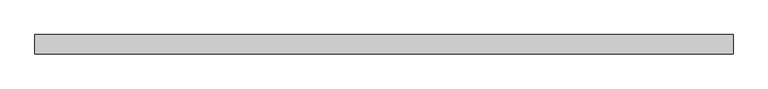
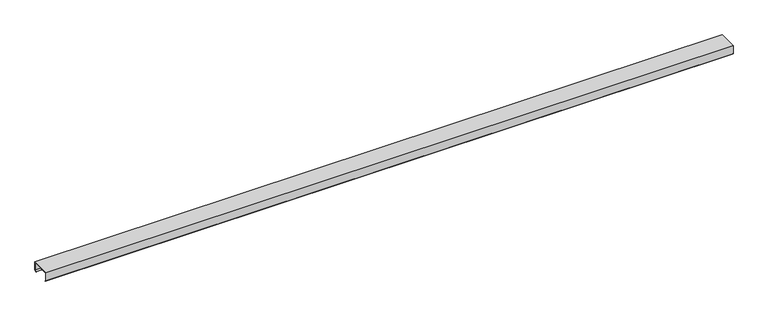
"""IFC4 building model written with IfcOpenShell, lengths in millimetres: proxy geometry, Generic Models 7:Generic Models 1:1:Generic Models 1:1 : Generic Models 7:Generic Models 1:337419:8 : Generic Models 7:Generic Models 1:1:Generic Models 1:1 : Generic Models 7:Generic Models 1:337419:306201."""

import ifcopenshell
import ifcopenshell.guid

model = None  # the IFC model being written
_history = None  # IfcOwnerHistory: only IFC2X3 demands one
_inside = {}  # id of a spatial element -> (the spatial element, [elements in it])
_under = {}  # id of a project, library or spatial element -> (it, [spatial elements below it])
_declared = {}  # id of a project -> (the project, [libraries it declares])
_typed = {}  # id of a type object -> (the type object, [elements of that type])
_made_of = {}  # id of a material, layer set ... -> (it, [elements and type objects made of it])


def new_model(schema):
    """Start an empty IFC model of exactly this schema.

    Asked for "IFC4X3", IfcOpenShell would pick the latest addendum, in which some entities
    have other attributes; the version numbers below select the first issue.
    IFC2X3 requires an IfcOwnerHistory on every rooted entity: one is made here for all.
    """
    global model, _history
    if schema == "IFC4X3":
        model = ifcopenshell.file(schema_version=(4, 3, 0, 0))
    else:
        model = ifcopenshell.file(schema=schema)
    _inside.clear()
    _under.clear()
    _declared.clear()
    _typed.clear()
    _made_of.clear()
    _history = None
    if model.schema == "IFC2X3":
        org = make("IfcOrganization", Name="unknown")
        user = make(
            "IfcPersonAndOrganization",
            ThePerson=make("IfcPerson", FamilyName="unknown"),
            TheOrganization=org,
        )
        app = make(
            "IfcApplication",
            ApplicationDeveloper=org,
            Version="unknown",
            ApplicationFullName="unknown",
            ApplicationIdentifier="unknown",
        )
        _history = make(
            "IfcOwnerHistory",
            OwningUser=user,
            OwningApplication=app,
            ChangeAction="ADDED",
            CreationDate=0,
        )
    return model


def make(cls, **values):
    """One entity of the class cls with the attributes given. An attribute that is None is left unset."""
    return model.create_entity(
        cls, **{name: value for name, value in values.items() if value is not None}
    )


def rooted(cls, **values):
    """An entity with a GlobalId (a new one), such as an element, a storey or a relation."""
    return make(cls, GlobalId=ifcopenshell.guid.new(), OwnerHistory=_history, **values)


def si_unit(unit_type, name, prefix=None):
    """IfcSIUnit, for example si_unit("LENGTHUNIT", "METRE", prefix="MILLI")."""
    return make("IfcSIUnit", UnitType=unit_type, Prefix=prefix, Name=name)


def assignment(units):
    """IfcUnitAssignment: the units of a project."""
    return None if units is None else make("IfcUnitAssignment", Units=units)


def point(xyz):
    """IfcCartesianPoint."""
    return None if xyz is None else make("IfcCartesianPoint", Coordinates=xyz)


def direction(xyz):
    """IfcDirection."""
    return None if xyz is None else make("IfcDirection", DirectionRatios=xyz)


def frame(location, z_axis=None, x_axis=None):
    """IfcAxis2Placement3D, a coordinate frame: its origin and axes. An axis left out is left unset."""
    return make(
        "IfcAxis2Placement3D",
        Location=point(location),
        Axis=direction(z_axis),
        RefDirection=direction(x_axis),
    )


def origin():
    """The frame at (0, 0, 0) with its axes left unset."""
    return frame((0.0, 0.0, 0.0))


def place(relative_to, where):
    """IfcLocalPlacement: puts the frame where relative to a parent placement (None: the world)."""
    return make(
        "IfcLocalPlacement", PlacementRelTo=relative_to, RelativePlacement=where
    )


def context(
    kind, dimensions, precision=None, world=None, true_north=None, identifier=None
):
    """IfcGeometricRepresentationContext, for example the 3D "Model" context."""
    return make(
        "IfcGeometricRepresentationContext",
        ContextIdentifier=identifier,
        ContextType=kind,
        CoordinateSpaceDimension=dimensions,
        Precision=precision,
        WorldCoordinateSystem=world,
        TrueNorth=true_north,
    )


def project(units=None, contexts=None):
    """IfcProject with its units and contexts."""
    return rooted(
        "IfcProject",
        Name="project",
        RepresentationContexts=contexts,
        UnitsInContext=assignment(units),
    )


def spatial(cls, under=None, at=None, **own):
    """A site, building, storey or space (cls), placed at a placement, below another one or the project."""
    s = rooted(cls, ObjectPlacement=at, **own)
    if under is not None:
        _under.setdefault(under.id(), (under, []))[1].append(s)
    return s


def polyline(points):
    """IfcPolyline through the points."""
    return make("IfcPolyline", Points=[point(p) for p in points])


def outline(outer, holes=None, kind="AREA"):
    """IfcArbitraryClosedProfileDef: a profile drawn as a closed curve; with holes, ...WithVoids."""
    if holes is None:
        return make("IfcArbitraryClosedProfileDef", ProfileType=kind, OuterCurve=outer)
    return make(
        "IfcArbitraryProfileDefWithVoids",
        ProfileType=kind,
        OuterCurve=outer,
        InnerCurves=holes,
    )


def extrude(swept, where, along, depth):
    """IfcExtrudedAreaSolid: the profile swept, set in the frame where, extruded along a direction by depth."""
    return make(
        "IfcExtrudedAreaSolid",
        SweptArea=swept,
        Position=where,
        ExtrudedDirection=direction(along),
        Depth=depth,
    )


def shape(context_of_items, identifier, shape_type, items):
    """IfcShapeRepresentation: the items that make up one representation, for example the "Body"."""
    return make(
        "IfcShapeRepresentation",
        ContextOfItems=context_of_items,
        RepresentationIdentifier=identifier,
        RepresentationType=shape_type,
        Items=items,
    )


def source(mapping_origin, context_of_items, identifier, shape_type, items):
    """IfcRepresentationMap: a shape defined once, which mapped items show again and again."""
    return make(
        "IfcRepresentationMap",
        MappingOrigin=mapping_origin,
        MappedRepresentation=shape(context_of_items, identifier, shape_type, items),
    )


def transform(
    local_origin,
    x_axis=None,
    y_axis=None,
    z_axis=None,
    scale=None,
    scale2=None,
    scale3=None,
    uniform=True,
):
    """IfcCartesianTransformationOperator3D, or its non-uniform kind. x_axis, y_axis, z_axis: its Axis1, 2, 3."""
    if uniform:
        return make(
            "IfcCartesianTransformationOperator3D",
            Axis1=direction(x_axis),
            Axis2=direction(y_axis),
            LocalOrigin=point(local_origin),
            Scale=scale,
            Axis3=direction(z_axis),
        )
    return make(
        "IfcCartesianTransformationOperator3DnonUniform",
        Axis1=direction(x_axis),
        Axis2=direction(y_axis),
        LocalOrigin=point(local_origin),
        Scale=scale,
        Axis3=direction(z_axis),
        Scale2=scale2,
        Scale3=scale3,
    )


def mapped(mapping_source, mapping_target):
    """IfcMappedItem: shows the shape of a source again, moved by a transform."""
    return make(
        "IfcMappedItem", MappingSource=mapping_source, MappingTarget=mapping_target
    )


def made_of(thing, what):
    """Note that an element or type object is made of a material, layer set ...; save() writes the relation."""
    if what is not None:
        _made_of.setdefault(what.id(), (what, []))[1].append(thing)
    return thing


def element(
    cls,
    number,
    at=None,
    inside=None,
    cuts=None,
    type_object=None,
    material=None,
    context=None,
    identifier="Body",
    shape_type=None,
    held_by="IfcProductDefinitionShape",
    body=None,
    shapes=None,
    **own,
):
    """One element of the class cls, such as IfcWall. Its Tag is "e" and its number.

    at: its placement. inside: the storey or other place that contains it. cuts: it is an
    opening in that element (IfcRelVoidsElement). A single representation is given by context,
    identifier, shape_type and body (its items); several are given by shapes. held_by: the class
    of the entity that holds the representations. save() writes the other relations.
    """
    e = rooted(cls, Tag="e%d" % number, ObjectPlacement=at, **own)
    if body is not None:
        shapes = [shape(context, identifier, shape_type, body)]
    if shapes is not None:
        e.Representation = make(held_by, Representations=shapes)
    if inside is not None:
        _inside.setdefault(inside.id(), (inside, []))[1].append(e)
    if cuts is not None:
        rooted(
            "IfcRelVoidsElement", RelatingBuildingElement=cuts, RelatedOpeningElement=e
        )
    if type_object is not None:
        _typed.setdefault(type_object.id(), (type_object, []))[1].append(e)
    return made_of(e, material)


def aggregate(whole, parts):
    """IfcRelAggregates: a whole, such as a stair, and the parts it consists of."""
    return rooted("IfcRelAggregates", RelatingObject=whole, RelatedObjects=parts)


def save(model, path):
    """Write the relations noted so far, then the file.

    IfcRelAggregates (storeys below a building ...), IfcRelContainedInSpatialStructure (elements
    in a storey), IfcRelDefinesByType, IfcRelAssociatesMaterial and IfcRelDeclares: one each for
    every whole, place, type object, material and project.
    """
    for whole, parts in _under.values():
        aggregate(whole, parts)
    for where, things in _inside.values():
        rooted(
            "IfcRelContainedInSpatialStructure",
            RelatedElements=things,
            RelatingStructure=where,
        )
    for kind, things in _typed.values():
        rooted("IfcRelDefinesByType", RelatedObjects=things, RelatingType=kind)
    for what, things in _made_of.values():
        rooted("IfcRelAssociatesMaterial", RelatedObjects=things, RelatingMaterial=what)
    for by, libraries in _declared.values():
        rooted("IfcRelDeclares", RelatingContext=by, RelatedDefinitions=libraries)
    model.write(path)


def generic_models_5b39e394(model_context):
    return source(origin(), model_context, "Body", "SweptSolid", [
        extrude(outline(polyline([(-579000.6913841, 4985.940625), (-578797.4913841, 4985.940625), (-578797.4913841, 4897.040625), (-578812.0845307, 4884.7955211), (-578813.8702751, 4886.9236883), (-578800.2695091, 4898.336086), (-578800.2695091, 4983.1625), (-578997.9132591, 4983.1625), (-578997.9132591, 4898.336086), (-578984.3124931, 4886.9236883), (-578986.0982375, 4884.7955211), (-579000.6913841, 4897.040625), (-579000.6913841, 4985.940625)])), frame((565582.1867239, 0.0, 0.0), z_axis=(1.0, 0.0, 0.0), x_axis=(0.0, 1.0, 0.0)), (0.0, 0.0, 1.0), 7315.2),
    ])


if __name__ == "__main__":
    model = new_model("IFC4")
    model_context = context("Model", 3, world=origin())
    ifc_project = project(units=[si_unit("LENGTHUNIT", "METRE", prefix="MILLI")], contexts=[model_context])
    site = spatial("IfcSite", under=ifc_project)
    building = spatial("IfcBuilding", under=site)
    placement = place(None, origin())
    generic_models_shape = generic_models_5b39e394(model_context)
    element("IfcBuildingElementProxy", 1, Name="Generic Models 7:Generic Models 1:1:Generic Models 1:1 : Generic Models 7:Generic Models 1:337419:8 : Generic Models 7:Generic Models 1:1:Generic Models 1:1 : Generic Models 7:Generic Models 1:337419:306201", ObjectType="Generic Models 7:Generic Models 1:1:Generic Models 1:1 : Generic Models 7:Generic Models 1:337419:8 : Generic Models 7:Generic Models 1:1:Generic Models 1:1 : Generic Models 7:Generic Models 1:337419:306201", at=placement, inside=building, context=model_context, shape_type="MappedRepresentation", body=[
        mapped(generic_models_shape, transform((0.0, 0.0, 0.0), x_axis=(1.0, 0.0, 0.0), y_axis=(0.0, 1.0, 0.0), z_axis=(0.0, 0.0, 1.0))),
    ])
    save(model, "model.ifc")

# Revit data of these elements
# Type "Generic Models 7:Generic Models 1:1:Generic Models 1:1 : Generic Models 7:Generic Models 1:337419:8 : Generic Models 7:Generic Models 1:1:Generic Models 1:1 : Generic Models 7:Generic Models 1:337419:306201"
#   NameOverride = "Generic Models 7:Generic Models 1:1:Generic Models 1:1 : Generic Models 7:Generic Models 1:337419:306201"
#   ObjectTypeOverride = "Generic Models 1:1 : Generic Models 7:Generic Models 1:337419"
#   Reference = "Generic Models 1"
#   Tag = "306201"
# Element 1 (IfcBuildingElementProxy, "Generic Models 7:Generic Models 1:1:Generic Models 1:1 : Generic Models 7:Generic Models 1:337419:8 : Generic Models 7:Generic Models 1:1:Generic Models 1:1 : Generic Models 7:Generic Models 1:337419:306201")
#   Materials on its faces: "CEE' SECTION (8.0x3.5C - SEE STRUCT. DWGS)"
# Materials
#   "CEE' SECTION (8.0x3.5C - SEE STRUCT. DWGS)": class "Unassigned", colour RGB 210 209 208, transparency 0, Keynote = "M05121300.02", Cost = 0
